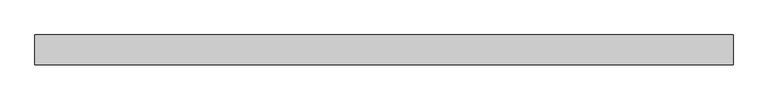
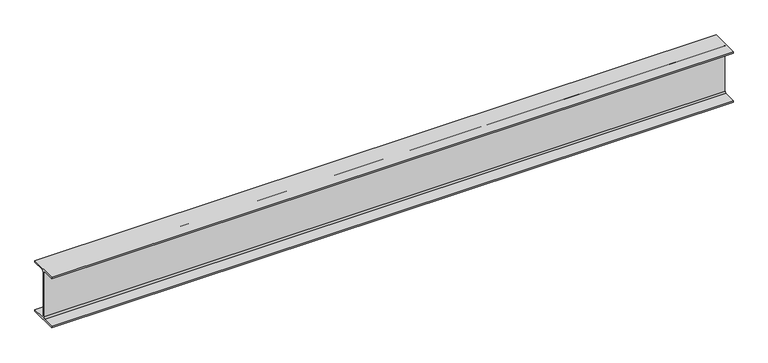
"""IFC4 building model written with IfcOpenShell, lengths in millimetres: beam geometry, Steel Beam_H-KSD3502 : H_SB_ASB_H-250x125x6x9."""

import ifcopenshell
import ifcopenshell.guid

model = None  # the IFC model being written
_history = None  # IfcOwnerHistory: only IFC2X3 demands one
_inside = {}  # id of a spatial element -> (the spatial element, [elements in it])
_under = {}  # id of a project, library or spatial element -> (it, [spatial elements below it])
_declared = {}  # id of a project -> (the project, [libraries it declares])
_typed = {}  # id of a type object -> (the type object, [elements of that type])
_made_of = {}  # id of a material, layer set ... -> (it, [elements and type objects made of it])


def new_model(schema):
    """Start an empty IFC model of exactly this schema.

    Asked for "IFC4X3", IfcOpenShell would pick the latest addendum, in which some entities
    have other attributes; the version numbers below select the first issue.
    IFC2X3 requires an IfcOwnerHistory on every rooted entity: one is made here for all.
    """
    global model, _history
    if schema == "IFC4X3":
        model = ifcopenshell.file(schema_version=(4, 3, 0, 0))
    else:
        model = ifcopenshell.file(schema=schema)
    _inside.clear()
    _under.clear()
    _declared.clear()
    _typed.clear()
    _made_of.clear()
    _history = None
    if model.schema == "IFC2X3":
        org = make("IfcOrganization", Name="unknown")
        user = make(
            "IfcPersonAndOrganization",
            ThePerson=make("IfcPerson", FamilyName="unknown"),
            TheOrganization=org,
        )
        app = make(
            "IfcApplication",
            ApplicationDeveloper=org,
            Version="unknown",
            ApplicationFullName="unknown",
            ApplicationIdentifier="unknown",
        )
        _history = make(
            "IfcOwnerHistory",
            OwningUser=user,
            OwningApplication=app,
            ChangeAction="ADDED",
            CreationDate=0,
        )
    return model


def make(cls, **values):
    """One entity of the class cls with the attributes given. An attribute that is None is left unset."""
    return model.create_entity(
        cls, **{name: value for name, value in values.items() if value is not None}
    )


def rooted(cls, **values):
    """An entity with a GlobalId (a new one), such as an element, a storey or a relation."""
    return make(cls, GlobalId=ifcopenshell.guid.new(), OwnerHistory=_history, **values)


def si_unit(unit_type, name, prefix=None):
    """IfcSIUnit, for example si_unit("LENGTHUNIT", "METRE", prefix="MILLI")."""
    return make("IfcSIUnit", UnitType=unit_type, Prefix=prefix, Name=name)


def assignment(units):
    """IfcUnitAssignment: the units of a project."""
    return None if units is None else make("IfcUnitAssignment", Units=units)


def point(xyz):
    """IfcCartesianPoint."""
    return None if xyz is None else make("IfcCartesianPoint", Coordinates=xyz)


def direction(xyz):
    """IfcDirection."""
    return None if xyz is None else make("IfcDirection", DirectionRatios=xyz)


def frame(location, z_axis=None, x_axis=None):
    """IfcAxis2Placement3D, a coordinate frame: its origin and axes. An axis left out is left unset."""
    return make(
        "IfcAxis2Placement3D",
        Location=point(location),
        Axis=direction(z_axis),
        RefDirection=direction(x_axis),
    )


def frame_2d(location, x_axis=None):
    """IfcAxis2Placement2D, a coordinate frame in the plane: its origin and x axis."""
    return make(
        "IfcAxis2Placement2D", Location=point(location), RefDirection=direction(x_axis)
    )


def origin():
    """The frame at (0, 0, 0) with its axes left unset."""
    return frame((0.0, 0.0, 0.0))


def place(relative_to, where):
    """IfcLocalPlacement: puts the frame where relative to a parent placement (None: the world)."""
    return make(
        "IfcLocalPlacement", PlacementRelTo=relative_to, RelativePlacement=where
    )


def context(
    kind, dimensions, precision=None, world=None, true_north=None, identifier=None
):
    """IfcGeometricRepresentationContext, for example the 3D "Model" context."""
    return make(
        "IfcGeometricRepresentationContext",
        ContextIdentifier=identifier,
        ContextType=kind,
        CoordinateSpaceDimension=dimensions,
        Precision=precision,
        WorldCoordinateSystem=world,
        TrueNorth=true_north,
    )


def project(units=None, contexts=None):
    """IfcProject with its units and contexts."""
    return rooted(
        "IfcProject",
        Name="project",
        RepresentationContexts=contexts,
        UnitsInContext=assignment(units),
    )


def spatial(cls, under=None, at=None, **own):
    """A site, building, storey or space (cls), placed at a placement, below another one or the project."""
    s = rooted(cls, ObjectPlacement=at, **own)
    if under is not None:
        _under.setdefault(under.id(), (under, []))[1].append(s)
    return s


def polyline(points):
    """IfcPolyline through the points."""
    return make("IfcPolyline", Points=[point(p) for p in points])


def circle_curve(where, radius):
    """IfcCircle in the frame where."""
    return make("IfcCircle", Position=where, Radius=radius)


def trimmed(basis, trim1, trim2, sense, master):
    """IfcTrimmedCurve: the piece of a basis curve between two trims."""
    return make(
        "IfcTrimmedCurve",
        BasisCurve=basis,
        Trim1=trim1,
        Trim2=trim2,
        SenseAgreement=sense,
        MasterRepresentation=master,
    )


def segment(curve, same_sense, transition):
    """IfcCompositeCurveSegment."""
    return make(
        "IfcCompositeCurveSegment",
        Transition=transition,
        SameSense=same_sense,
        ParentCurve=curve,
    )


def composite_curve(segments, self_intersect=None):
    """IfcCompositeCurve: segments joined end to end."""
    return make("IfcCompositeCurve", Segments=segments, SelfIntersect=self_intersect)


def outline(outer, holes=None, kind="AREA"):
    """IfcArbitraryClosedProfileDef: a profile drawn as a closed curve; with holes, ...WithVoids."""
    if holes is None:
        return make("IfcArbitraryClosedProfileDef", ProfileType=kind, OuterCurve=outer)
    return make(
        "IfcArbitraryProfileDefWithVoids",
        ProfileType=kind,
        OuterCurve=outer,
        InnerCurves=holes,
    )


def extrude(swept, where, along, depth):
    """IfcExtrudedAreaSolid: the profile swept, set in the frame where, extruded along a direction by depth."""
    return make(
        "IfcExtrudedAreaSolid",
        SweptArea=swept,
        Position=where,
        ExtrudedDirection=direction(along),
        Depth=depth,
    )


def shape(context_of_items, identifier, shape_type, items):
    """IfcShapeRepresentation: the items that make up one representation, for example the "Body"."""
    return make(
        "IfcShapeRepresentation",
        ContextOfItems=context_of_items,
        RepresentationIdentifier=identifier,
        RepresentationType=shape_type,
        Items=items,
    )


def source(mapping_origin, context_of_items, identifier, shape_type, items):
    """IfcRepresentationMap: a shape defined once, which mapped items show again and again."""
    return make(
        "IfcRepresentationMap",
        MappingOrigin=mapping_origin,
        MappedRepresentation=shape(context_of_items, identifier, shape_type, items),
    )


def transform(
    local_origin,
    x_axis=None,
    y_axis=None,
    z_axis=None,
    scale=None,
    scale2=None,
    scale3=None,
    uniform=True,
):
    """IfcCartesianTransformationOperator3D, or its non-uniform kind. x_axis, y_axis, z_axis: its Axis1, 2, 3."""
    if uniform:
        return make(
            "IfcCartesianTransformationOperator3D",
            Axis1=direction(x_axis),
            Axis2=direction(y_axis),
            LocalOrigin=point(local_origin),
            Scale=scale,
            Axis3=direction(z_axis),
        )
    return make(
        "IfcCartesianTransformationOperator3DnonUniform",
        Axis1=direction(x_axis),
        Axis2=direction(y_axis),
        LocalOrigin=point(local_origin),
        Scale=scale,
        Axis3=direction(z_axis),
        Scale2=scale2,
        Scale3=scale3,
    )


def mapped(mapping_source, mapping_target):
    """IfcMappedItem: shows the shape of a source again, moved by a transform."""
    return make(
        "IfcMappedItem", MappingSource=mapping_source, MappingTarget=mapping_target
    )


def made_of(thing, what):
    """Note that an element or type object is made of a material, layer set ...; save() writes the relation."""
    if what is not None:
        _made_of.setdefault(what.id(), (what, []))[1].append(thing)
    return thing


def element(
    cls,
    number,
    at=None,
    inside=None,
    cuts=None,
    type_object=None,
    material=None,
    context=None,
    identifier="Body",
    shape_type=None,
    held_by="IfcProductDefinitionShape",
    body=None,
    shapes=None,
    **own,
):
    """One element of the class cls, such as IfcWall. Its Tag is "e" and its number.

    at: its placement. inside: the storey or other place that contains it. cuts: it is an
    opening in that element (IfcRelVoidsElement). A single representation is given by context,
    identifier, shape_type and body (its items); several are given by shapes. held_by: the class
    of the entity that holds the representations. save() writes the other relations.
    """
    e = rooted(cls, Tag="e%d" % number, ObjectPlacement=at, **own)
    if body is not None:
        shapes = [shape(context, identifier, shape_type, body)]
    if shapes is not None:
        e.Representation = make(held_by, Representations=shapes)
    if inside is not None:
        _inside.setdefault(inside.id(), (inside, []))[1].append(e)
    if cuts is not None:
        rooted(
            "IfcRelVoidsElement", RelatingBuildingElement=cuts, RelatedOpeningElement=e
        )
    if type_object is not None:
        _typed.setdefault(type_object.id(), (type_object, []))[1].append(e)
    return made_of(e, material)


def aggregate(whole, parts):
    """IfcRelAggregates: a whole, such as a stair, and the parts it consists of."""
    return rooted("IfcRelAggregates", RelatingObject=whole, RelatedObjects=parts)


def save(model, path):
    """Write the relations noted so far, then the file.

    IfcRelAggregates (storeys below a building ...), IfcRelContainedInSpatialStructure (elements
    in a storey), IfcRelDefinesByType, IfcRelAssociatesMaterial and IfcRelDeclares: one each for
    every whole, place, type object, material and project.
    """
    for whole, parts in _under.values():
        aggregate(whole, parts)
    for where, things in _inside.values():
        rooted(
            "IfcRelContainedInSpatialStructure",
            RelatedElements=things,
            RelatingStructure=where,
        )
    for kind, things in _typed.values():
        rooted("IfcRelDefinesByType", RelatedObjects=things, RelatingType=kind)
    for what, things in _made_of.values():
        rooted("IfcRelAssociatesMaterial", RelatedObjects=things, RelatingMaterial=what)
    for by, libraries in _declared.values():
        rooted("IfcRelDeclares", RelatingContext=by, RelatedDefinitions=libraries)
    model.write(path)


def beam_4107c911(model_context):
    return source(origin(), model_context, "Body", "SweptSolid", [
        extrude(outline(composite_curve([segment(polyline([(82.5, -141.5), (82.5, -151.7), (-82.5, -151.7), (-82.5, -141.5), (-11.9, -141.5)]), True, "CONTINUOUS"), segment(trimmed(circle_curve(frame_2d((-11.9, -132.6)), 8.9), [point((-11.9, -141.5))], [point((-3.0, -132.6))], True, "CARTESIAN"), True, "CONTINUOUS"), segment(polyline([(-3.0, -132.6), (-3.0, 132.6)]), True, "CONTINUOUS"), segment(trimmed(circle_curve(frame_2d((-11.9, 132.6)), 8.9), [point((-3.0, 132.6))], [point((-11.9, 141.5))], True, "CARTESIAN"), True, "CONTINUOUS"), segment(polyline([(-11.9, 141.5), (-82.5, 141.5), (-82.5, 151.7), (82.5, 151.7), (82.5, 141.5), (11.9, 141.5)]), True, "CONTINUOUS"), segment(trimmed(circle_curve(frame_2d((11.9, 132.6)), 8.9), [point((11.9, 141.5))], [point((3.0, 132.6))], True, "CARTESIAN"), True, "CONTINUOUS"), segment(polyline([(3.0, 132.6), (3.0, -132.6)]), True, "CONTINUOUS"), segment(trimmed(circle_curve(frame_2d((11.9, -132.6)), 8.9), [point((3.0, -132.6))], [point((11.9, -141.5))], True, "CARTESIAN"), True, "CONTINUOUS"), segment(polyline([(11.9, -141.5), (82.5, -141.5)]), True, "CONTINUOUS")], self_intersect=False)), frame((-1830.0827532, 0.0, 0.0), z_axis=(1.0, 0.0, 0.0), x_axis=(0.0, 1.0, 0.0)), (0.0, 0.0, 1.0), 3859.8827532),
    ])


if __name__ == "__main__":
    model = new_model("IFC4")
    model_context = context("Model", 3, world=origin())
    ifc_project = project(units=[si_unit("LENGTHUNIT", "METRE", prefix="MILLI")], contexts=[model_context])
    site = spatial("IfcSite", under=ifc_project)
    building = spatial("IfcBuilding", under=site)
    placement = place(None, origin())
    beam_shape = beam_4107c911(model_context)
    element("IfcBeam", 1, ObjectType="Steel Beam_H-KSD3502 : H_SB_ASB_H-250x125x6x9", at=placement, inside=building, context=model_context, shape_type="MappedRepresentation", body=[
        mapped(beam_shape, transform((0.0, 0.0, 0.0), x_axis=(1.0, 0.0, 0.0), y_axis=(0.0, 1.0, 0.0), z_axis=(0.0, 0.0, 1.0))),
    ])
    save(model, "model.ifc")

# Revit data of these elements
# Type "Steel Beam_H-KSD3502 : H_SB_ASB_H-250x125x6x9"
#   Width = 12.5 cm
#   Web Thickness = 0.6 cm
#   Web Fillet = 1.2 cm
#   Warping Constant = 42539.8 cm⁶
#   Torsional Moment of Inertia = 7.8102 cm⁴
#   Torsional Modulus = 1.0 cm³
#   Section Area = 37.66 cm²
#   Plastic Modulus weak axis = 73.1 cm³
#   Plastic Modulus strong axis = 366.0 cm³
#   Perimeter = 0.97 m²/m
#   Nominal Weight = 29.60 kgf/m
#   Moment of Inertia weak axis = 294.00 cm⁴
#   Moment of Inertia strong axis = 4050.00 cm⁴
#   Height = 25.0 cm
#   Flange Thickness = 0.9 cm
#   Elastic Modulus weak axis = 47.0 cm³
#   Elastic Modulus strong axis = 324.0 cm³
#   Centroid Vertical = 12.5 cm
#   Centroid Horizontal = 6.25 cm
#   Length [instance default] = 1.5240 m
#   Structural Material [instance default] = Steel, 45-345
#   Assembly Code = ""
# Element 1 (IfcBeam, "Steel Beam_H-KSD3502 : H_SB_ASB_H-250x125x6x9")
#   Structural Material = none
# Materials
#   "Steel, 45-345": class "Metal", colour RGB 189 187 185, transparency 0, Description = "Steel 345 MPa", Cost = 0
